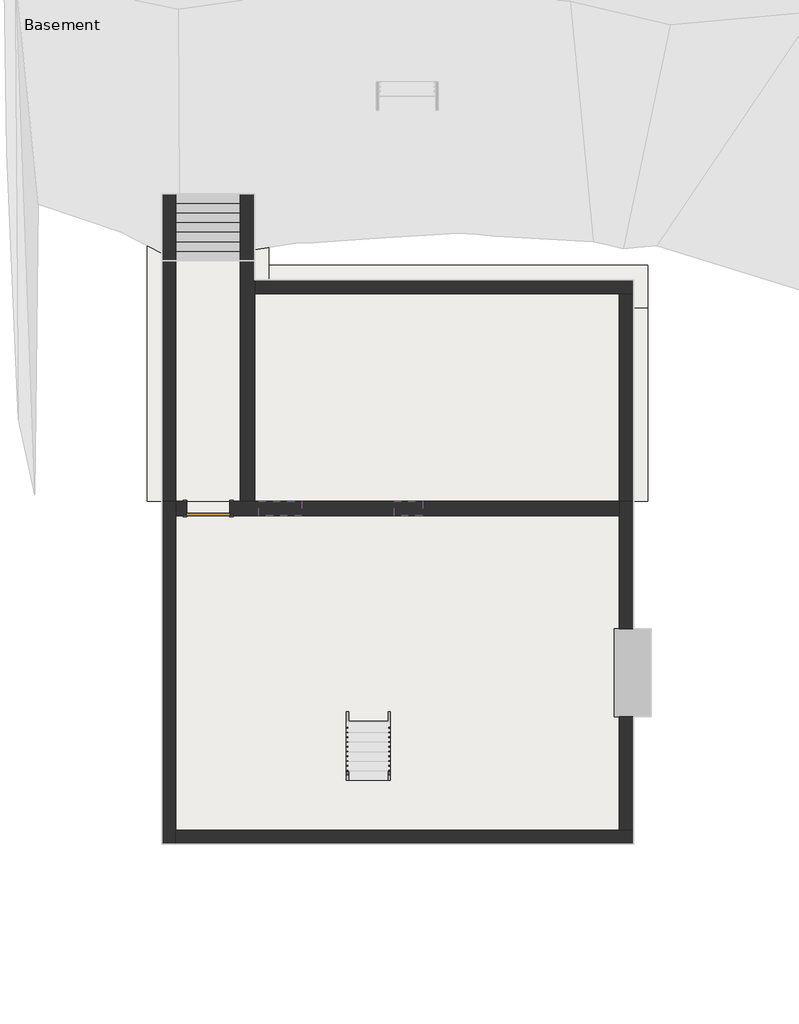
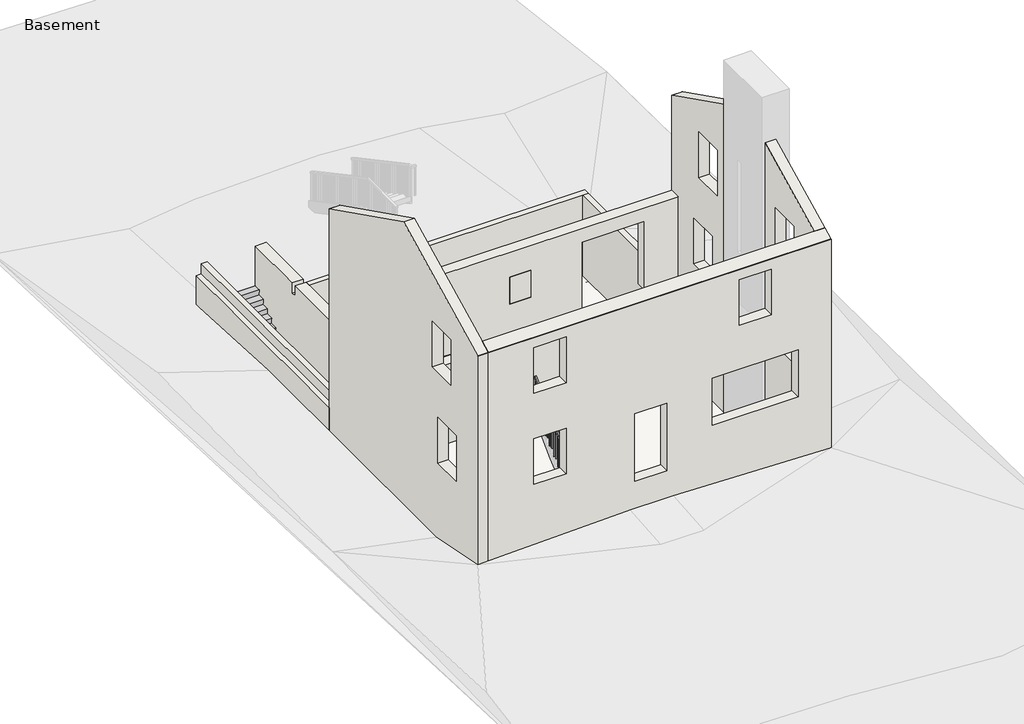
# One storey, part 1 of 2: 11 walls, 4 footings, 4 slabs, 2 railings, 1 door, 1 stair flight.
"""IFC4 building model written with IfcOpenShell, lengths in millimetres."""

import ifcopenshell
import ifcopenshell.guid

model = None  # the IFC model being written
_history = None  # IfcOwnerHistory: only IFC2X3 demands one
_inside = {}  # id of a spatial element -> (the spatial element, [elements in it])
_under = {}  # id of a project, library or spatial element -> (it, [spatial elements below it])
_declared = {}  # id of a project -> (the project, [libraries it declares])
_typed = {}  # id of a type object -> (the type object, [elements of that type])
_made_of = {}  # id of a material, layer set ... -> (it, [elements and type objects made of it])


def new_model(schema):
    """Start an empty IFC model of exactly this schema.

    Asked for "IFC4X3", IfcOpenShell would pick the latest addendum, in which some entities
    have other attributes; the version numbers below select the first issue.
    IFC2X3 requires an IfcOwnerHistory on every rooted entity: one is made here for all.
    """
    global model, _history
    if schema == "IFC4X3":
        model = ifcopenshell.file(schema_version=(4, 3, 0, 0))
    else:
        model = ifcopenshell.file(schema=schema)
    _inside.clear()
    _under.clear()
    _declared.clear()
    _typed.clear()
    _made_of.clear()
    _history = None
    if model.schema == "IFC2X3":
        org = make("IfcOrganization", Name="unknown")
        user = make(
            "IfcPersonAndOrganization",
            ThePerson=make("IfcPerson", FamilyName="unknown"),
            TheOrganization=org,
        )
        app = make(
            "IfcApplication",
            ApplicationDeveloper=org,
            Version="unknown",
            ApplicationFullName="unknown",
            ApplicationIdentifier="unknown",
        )
        _history = make(
            "IfcOwnerHistory",
            OwningUser=user,
            OwningApplication=app,
            ChangeAction="ADDED",
            CreationDate=0,
        )
    return model


def make(cls, **values):
    """One entity of the class cls with the attributes given. An attribute that is None is left unset."""
    return model.create_entity(
        cls, **{name: value for name, value in values.items() if value is not None}
    )


def rooted(cls, **values):
    """An entity with a GlobalId (a new one), such as an element, a storey or a relation."""
    return make(cls, GlobalId=ifcopenshell.guid.new(), OwnerHistory=_history, **values)


def si_unit(unit_type, name, prefix=None):
    """IfcSIUnit, for example si_unit("LENGTHUNIT", "METRE", prefix="MILLI")."""
    return make("IfcSIUnit", UnitType=unit_type, Prefix=prefix, Name=name)


def assignment(units):
    """IfcUnitAssignment: the units of a project."""
    return None if units is None else make("IfcUnitAssignment", Units=units)


def point(xyz):
    """IfcCartesianPoint."""
    return None if xyz is None else make("IfcCartesianPoint", Coordinates=xyz)


def direction(xyz):
    """IfcDirection."""
    return None if xyz is None else make("IfcDirection", DirectionRatios=xyz)


def frame(location, z_axis=None, x_axis=None):
    """IfcAxis2Placement3D, a coordinate frame: its origin and axes. An axis left out is left unset."""
    return make(
        "IfcAxis2Placement3D",
        Location=point(location),
        Axis=direction(z_axis),
        RefDirection=direction(x_axis),
    )


def origin():
    """The frame at (0, 0, 0) with its axes left unset."""
    return frame((0.0, 0.0, 0.0))


def origin_with_axes():
    """The frame at (0, 0, 0) with the z axis (0, 0, 1) and the x axis (1, 0, 0) written out."""
    return frame((0.0, 0.0, 0.0), z_axis=(0.0, 0.0, 1.0), x_axis=(1.0, 0.0, 0.0))


def place(relative_to, where):
    """IfcLocalPlacement: puts the frame where relative to a parent placement (None: the world)."""
    return make(
        "IfcLocalPlacement", PlacementRelTo=relative_to, RelativePlacement=where
    )


def context(
    kind, dimensions, precision=None, world=None, true_north=None, identifier=None
):
    """IfcGeometricRepresentationContext, for example the 3D "Model" context."""
    return make(
        "IfcGeometricRepresentationContext",
        ContextIdentifier=identifier,
        ContextType=kind,
        CoordinateSpaceDimension=dimensions,
        Precision=precision,
        WorldCoordinateSystem=world,
        TrueNorth=true_north,
    )


def project(units=None, contexts=None):
    """IfcProject with its units and contexts."""
    return rooted(
        "IfcProject",
        Name="project",
        RepresentationContexts=contexts,
        UnitsInContext=assignment(units),
    )


def spatial(cls, under=None, at=None, **own):
    """A site, building, storey or space (cls), placed at a placement, below another one or the project."""
    s = rooted(cls, ObjectPlacement=at, **own)
    if under is not None:
        _under.setdefault(under.id(), (under, []))[1].append(s)
    return s


def polyline(points):
    """IfcPolyline through the points."""
    return make("IfcPolyline", Points=[point(p) for p in points])


def outline(outer, holes=None, kind="AREA"):
    """IfcArbitraryClosedProfileDef: a profile drawn as a closed curve; with holes, ...WithVoids."""
    if holes is None:
        return make("IfcArbitraryClosedProfileDef", ProfileType=kind, OuterCurve=outer)
    return make(
        "IfcArbitraryProfileDefWithVoids",
        ProfileType=kind,
        OuterCurve=outer,
        InnerCurves=holes,
    )


def extrude(swept, where, along, depth):
    """IfcExtrudedAreaSolid: the profile swept, set in the frame where, extruded along a direction by depth."""
    return make(
        "IfcExtrudedAreaSolid",
        SweptArea=swept,
        Position=where,
        ExtrudedDirection=direction(along),
        Depth=depth,
    )


def faces_of(points, faces, orient=None, outer=None):
    """IfcFace entities. A face is a list of loops; a loop is a list of indices into points, from 0.

    orient and outer hold one flag for each loop. By default every Orientation is true, the
    first loop of a face is its IfcFaceOuterBound and the others are IfcFaceBound.
    """
    made = []
    for i, loops in enumerate(faces):
        bounds = []
        for j, loop in enumerate(loops):
            is_outer = j == 0 if outer is None else outer[i][j]
            bounds.append(
                make(
                    "IfcFaceOuterBound" if is_outer else "IfcFaceBound",
                    Bound=make("IfcPolyLoop", Polygon=[points[k] for k in loop]),
                    Orientation=True if orient is None else orient[i][j],
                )
            )
        made.append(make("IfcFace", Bounds=bounds))
    return made


def faceted_brep(points, faces, orient=None, outer=None, voids=None):
    """IfcFacetedBrep: a solid bounded by flat faces; with voids (closed shells), ...WithVoids."""
    shared = [point(p) for p in points]
    hull = make("IfcClosedShell", CfsFaces=faces_of(shared, faces, orient, outer))
    if voids is None:
        return make("IfcFacetedBrep", Outer=hull)
    return make(
        "IfcFacetedBrepWithVoids",
        Outer=hull,
        Voids=[
            make(cls, CfsFaces=faces_of(shared, fs, o, b)) for cls, fs, o, b in voids
        ],
    )


def shape(context_of_items, identifier, shape_type, items):
    """IfcShapeRepresentation: the items that make up one representation, for example the "Body"."""
    return make(
        "IfcShapeRepresentation",
        ContextOfItems=context_of_items,
        RepresentationIdentifier=identifier,
        RepresentationType=shape_type,
        Items=items,
    )


def source(mapping_origin, context_of_items, identifier, shape_type, items):
    """IfcRepresentationMap: a shape defined once, which mapped items show again and again."""
    return make(
        "IfcRepresentationMap",
        MappingOrigin=mapping_origin,
        MappedRepresentation=shape(context_of_items, identifier, shape_type, items),
    )


def transform(
    local_origin,
    x_axis=None,
    y_axis=None,
    z_axis=None,
    scale=None,
    scale2=None,
    scale3=None,
    uniform=True,
):
    """IfcCartesianTransformationOperator3D, or its non-uniform kind. x_axis, y_axis, z_axis: its Axis1, 2, 3."""
    if uniform:
        return make(
            "IfcCartesianTransformationOperator3D",
            Axis1=direction(x_axis),
            Axis2=direction(y_axis),
            LocalOrigin=point(local_origin),
            Scale=scale,
            Axis3=direction(z_axis),
        )
    return make(
        "IfcCartesianTransformationOperator3DnonUniform",
        Axis1=direction(x_axis),
        Axis2=direction(y_axis),
        LocalOrigin=point(local_origin),
        Scale=scale,
        Axis3=direction(z_axis),
        Scale2=scale2,
        Scale3=scale3,
    )


def mapped(mapping_source, mapping_target):
    """IfcMappedItem: shows the shape of a source again, moved by a transform."""
    return make(
        "IfcMappedItem", MappingSource=mapping_source, MappingTarget=mapping_target
    )


def made_of(thing, what):
    """Note that an element or type object is made of a material, layer set ...; save() writes the relation."""
    if what is not None:
        _made_of.setdefault(what.id(), (what, []))[1].append(thing)
    return thing


def element(
    cls,
    number,
    at=None,
    inside=None,
    cuts=None,
    type_object=None,
    material=None,
    context=None,
    identifier="Body",
    shape_type=None,
    held_by="IfcProductDefinitionShape",
    body=None,
    shapes=None,
    **own,
):
    """One element of the class cls, such as IfcWall. Its Tag is "e" and its number.

    at: its placement. inside: the storey or other place that contains it. cuts: it is an
    opening in that element (IfcRelVoidsElement). A single representation is given by context,
    identifier, shape_type and body (its items); several are given by shapes. held_by: the class
    of the entity that holds the representations. save() writes the other relations.
    """
    e = rooted(cls, Tag="e%d" % number, ObjectPlacement=at, **own)
    if body is not None:
        shapes = [shape(context, identifier, shape_type, body)]
    if shapes is not None:
        e.Representation = make(held_by, Representations=shapes)
    if inside is not None:
        _inside.setdefault(inside.id(), (inside, []))[1].append(e)
    if cuts is not None:
        rooted(
            "IfcRelVoidsElement", RelatingBuildingElement=cuts, RelatedOpeningElement=e
        )
    if type_object is not None:
        _typed.setdefault(type_object.id(), (type_object, []))[1].append(e)
    return made_of(e, material)


def aggregate(whole, parts):
    """IfcRelAggregates: a whole, such as a stair, and the parts it consists of."""
    return rooted("IfcRelAggregates", RelatingObject=whole, RelatedObjects=parts)


def save(model, path):
    """Write the relations noted so far, then the file.

    IfcRelAggregates (storeys below a building ...), IfcRelContainedInSpatialStructure (elements
    in a storey), IfcRelDefinesByType, IfcRelAssociatesMaterial and IfcRelDeclares: one each for
    every whole, place, type object, material and project.
    """
    for whole, parts in _under.values():
        aggregate(whole, parts)
    for where, things in _inside.values():
        rooted(
            "IfcRelContainedInSpatialStructure",
            RelatedElements=things,
            RelatingStructure=where,
        )
    for kind, things in _typed.values():
        rooted("IfcRelDefinesByType", RelatedObjects=things, RelatingType=kind)
    for what, things in _made_of.values():
        rooted("IfcRelAssociatesMaterial", RelatedObjects=things, RelatingMaterial=what)
    for by, libraries in _declared.values():
        rooted("IfcRelDeclares", RelatingContext=by, RelatedDefinitions=libraries)
    model.write(path)


def door_03272193(model_context):
    return source(origin(), model_context, "Body", "SweptSolid", [
        extrude(outline(polyline([(2209.8, -533.4), (0.0, -533.4), (0.0, -457.2), (2133.6, -457.2), (2133.6, 457.2), (0.0, 457.2), (0.0, 533.4), (2209.8, 533.4), (2209.8, -533.4)])), frame((0.0, 152.4, 0.0), z_axis=(0.0, 1.0, 0.0), x_axis=(0.0, 0.0, 1.0)), (0.0, 0.0, 1.0), 25.4),
        extrude(outline(polyline([(2209.8, 533.4), (2209.8, -533.4), (0.0, -533.4), (0.0, -457.2), (2133.6, -457.2), (2133.6, 457.2), (0.0, 457.2), (0.0, 533.4), (2209.8, 533.4)])), frame((0.0, -177.8, 0.0), z_axis=(0.0, 1.0, 0.0), x_axis=(0.0, 0.0, 1.0)), (0.0, 0.0, 1.0), 25.4),
        extrude(outline(polyline([(457.2, 101.6), (-457.2, 101.6), (-457.2, 152.4), (457.2, 152.4), (457.2, 101.6)])), origin_with_axes(), (0.0, 0.0, 1.0), 2133.6),
    ])


model = new_model("IFC4")

# Units and contexts
model_context = context("Model", 3, world=origin())
ifc_project = project(units=[si_unit("LENGTHUNIT", "METRE", prefix="MILLI")], contexts=[model_context])

# Site, building, storey
site = spatial("IfcSite", under=ifc_project)
building = spatial("IfcBuilding", under=site)
storey = spatial("IfcBuildingStorey", under=building, Name="Basement", Elevation=-2667.0)

# Door
placement = place(None, origin())
door_shape = door_03272193(model_context)
element("IfcDoor", 1, ObjectType="Single-Flush : 36\" x 84\"", at=placement, inside=storey, context=model_context, shape_type="MappedRepresentation", body=[
    mapped(door_shape, transform((-4998.5803068, 2999.6888758, -2667.0), x_axis=(-1.0, 0.0, 0.0), y_axis=(0.0, -1.0, 0.0), z_axis=(0.0, 0.0, 1.0))),
])

# Footings
element("IfcFooting", 2, ObjectType="Bearing Footing - 36\" x 12\"", at=placement, inside=storey, context=model_context, shape_type="SweptSolid", body=[
    extrude(outline(polyline([(-5379.5803068, 3152.0888758), (-6293.9803068, 3152.0888758), (-6293.9803068, 10010.0888758), (-5379.5803068, 10010.0888758), (-5379.5803068, 3152.0888758)])), frame((0.0, 0.0, -3073.4), z_axis=(0.0, 0.0, 1.0), x_axis=(1.0, 0.0, 0.0)), (0.0, 0.0, 1.0), 304.8),
])
element("IfcFooting", 3, ObjectType="Bearing Footing - 36\" x 12\"", at=placement, inside=storey, context=model_context, shape_type="Brep", body=[
    faceted_brep([(-3703.1803068, 7266.8888758, -2768.6), (3459.6196932, 7266.8888758, -2768.6), (4374.0196932, 7266.8888758, -2768.6), (4374.0196932, 8181.2888758, -2768.6), (-3703.1803068, 8181.2888758, -2768.6), (-3703.1803068, 8181.2888758, -3073.4), (4374.0196932, 8181.2888758, -3073.4), (-3703.1803068, 7266.8888758, -3073.4), (4374.0196932, 7266.8888758, -3073.4), (3459.6196932, 7266.8888758, -3073.4)], [[[0, 1, 2, 3, 4]], [[5, 4, 3, 6]], [[7, 5, 6, 8, 9]], [[0, 7, 9, 8, 2, 1]], [[0, 4, 5, 7]], [[3, 2, 8, 6]]]),
])
element("IfcFooting", 4, ObjectType="Bearing Footing - 36\" x 12\"", at=placement, inside=storey, context=model_context, shape_type="SweptSolid", body=[
    extrude(outline(polyline([(4374.0196932, 3152.0888758), (3459.6196932, 3152.0888758), (3459.6196932, 7266.8888758), (4374.0196932, 7266.8888758), (4374.0196932, 3152.0888758)])), frame((0.0, 0.0, -3073.4), z_axis=(0.0, 0.0, 1.0), x_axis=(1.0, 0.0, 0.0)), (0.0, 0.0, 1.0), 304.8),
])
element("IfcFooting", 5, ObjectType="Bearing Footing - 36\" x 12\"", at=placement, inside=storey, context=model_context, shape_type="Brep", body=[
    faceted_brep([(-3703.1803068, 3152.0888758, -2768.6), (-4617.5803068, 3152.0888758, -2768.6), (-4617.5803068, 3152.0888758, -3073.4), (-3703.1803068, 3152.0888758, -3073.4), (-4617.5803068, 10010.0888758, -2768.6), (-3703.1803068, 10010.0888758, -2768.6), (-3703.1803068, 10010.0888758, -3073.4), (-4617.5803068, 10010.0888758, -3073.4), (-3703.1803068, 7266.8888758, -2768.6), (-3703.1803068, 8181.2888758, -2768.6), (-3703.1803068, 8181.2888758, -3073.4), (-3703.1803068, 7266.8888758, -3073.4)], [[[0, 1, 2, 3]], [[4, 5, 6, 7]], [[0, 8, 9, 5, 4, 1]], [[2, 1, 4, 7]], [[3, 2, 7, 6, 10, 11]], [[0, 3, 11, 10, 6, 5, 9, 8]]]),
])

# Railings
element("IfcRailing", 6, ObjectType="Handrail - Rectangular", at=placement, inside=storey, context=model_context, shape_type="SweptSolid", body=[
    extrude(outline(polyline([(-2791.5111242, -1631.7331862), (-2791.5111242, -1562.1), (-149.9111242, 914.4), (-149.9111242, 844.7668138), (-2791.5111242, -1631.7331862)])), frame((-1163.1803068, 0.0, 0.0), z_axis=(1.0, 0.0, 0.0), x_axis=(0.0, 1.0, 0.0)), (0.0, 0.0, 1.0), 50.8),
    extrude(outline(polyline([(-261.0361242, 740.5871263), (-241.9861242, 758.4465013), (-241.9861242, -190.5), (-261.0361242, -190.5), (-261.0361242, 740.5871263)])), frame((-1147.3053068, 0.0, 0.0), z_axis=(1.0, 0.0, 0.0), x_axis=(0.0, 1.0, 0.0)), (0.0, 0.0, 1.0), 19.05),
    extrude(outline(polyline([(-362.6361242, 645.3371263), (-343.5861242, 663.1965013), (-343.5861242, -190.5), (-362.6361242, -190.5), (-362.6361242, 645.3371263)])), frame((-1147.3053068, 0.0, 0.0), z_axis=(1.0, 0.0, 0.0), x_axis=(0.0, 1.0, 0.0)), (0.0, 0.0, 1.0), 19.05),
    extrude(outline(polyline([(-464.2361242, 550.0871263), (-445.1861242, 567.9465013), (-445.1861242, -381.0), (-464.2361242, -381.0), (-464.2361242, 550.0871263)])), frame((-1147.3053068, 0.0, 0.0), z_axis=(1.0, 0.0, 0.0), x_axis=(0.0, 1.0, 0.0)), (0.0, 0.0, 1.0), 19.05),
    extrude(outline(polyline([(-565.8361242, 454.8371263), (-546.7861242, 472.6965013), (-546.7861242, -381.0), (-565.8361242, -381.0), (-565.8361242, 454.8371263)])), frame((-1147.3053068, 0.0, 0.0), z_axis=(1.0, 0.0, 0.0), x_axis=(0.0, 1.0, 0.0)), (0.0, 0.0, 1.0), 19.05),
    extrude(outline(polyline([(-667.4361242, 359.5871263), (-648.3861242, 377.4465013), (-648.3861242, -571.5), (-667.4361242, -571.5), (-667.4361242, 359.5871263)])), frame((-1147.3053068, 0.0, 0.0), z_axis=(1.0, 0.0, 0.0), x_axis=(0.0, 1.0, 0.0)), (0.0, 0.0, 1.0), 19.05),
    extrude(outline(polyline([(-769.0361242, 264.3371263), (-749.9861242, 282.1965013), (-749.9861242, -571.5), (-769.0361242, -571.5), (-769.0361242, 264.3371263)])), frame((-1147.3053068, 0.0, 0.0), z_axis=(1.0, 0.0, 0.0), x_axis=(0.0, 1.0, 0.0)), (0.0, 0.0, 1.0), 19.05),
    extrude(outline(polyline([(-870.6361242, 169.0871263), (-851.5861242, 186.9465013), (-851.5861242, -762.0), (-870.6361242, -762.0), (-870.6361242, 169.0871263)])), frame((-1147.3053068, 0.0, 0.0), z_axis=(1.0, 0.0, 0.0), x_axis=(0.0, 1.0, 0.0)), (0.0, 0.0, 1.0), 19.05),
    extrude(outline(polyline([(-972.2361242, 73.8371263), (-953.1861242, 91.6965013), (-953.1861242, -762.0), (-972.2361242, -762.0), (-972.2361242, 73.8371263)])), frame((-1147.3053068, 0.0, 0.0), z_axis=(1.0, 0.0, 0.0), x_axis=(0.0, 1.0, 0.0)), (0.0, 0.0, 1.0), 19.05),
    extrude(outline(polyline([(-1073.8361242, -21.4128737), (-1054.7861242, -3.5534987), (-1054.7861242, -952.5), (-1073.8361242, -952.5), (-1073.8361242, -21.4128737)])), frame((-1147.3053068, 0.0, 0.0), z_axis=(1.0, 0.0, 0.0), x_axis=(0.0, 1.0, 0.0)), (0.0, 0.0, 1.0), 19.05),
    extrude(outline(polyline([(-1175.4361242, -116.6628737), (-1156.3861242, -98.8034987), (-1156.3861242, -952.5), (-1175.4361242, -952.5), (-1175.4361242, -116.6628737)])), frame((-1147.3053068, 0.0, 0.0), z_axis=(1.0, 0.0, 0.0), x_axis=(0.0, 1.0, 0.0)), (0.0, 0.0, 1.0), 19.05),
    extrude(outline(polyline([(-1277.0361242, -211.9128737), (-1257.9861242, -194.0534987), (-1257.9861242, -1143.0), (-1277.0361242, -1143.0), (-1277.0361242, -211.9128737)])), frame((-1147.3053068, 0.0, 0.0), z_axis=(1.0, 0.0, 0.0), x_axis=(0.0, 1.0, 0.0)), (0.0, 0.0, 1.0), 19.05),
    extrude(outline(polyline([(-1378.6361242, -307.1628737), (-1359.5861242, -289.3034987), (-1359.5861242, -1143.0), (-1378.6361242, -1143.0), (-1378.6361242, -307.1628737)])), frame((-1147.3053068, 0.0, 0.0), z_axis=(1.0, 0.0, 0.0), x_axis=(0.0, 1.0, 0.0)), (0.0, 0.0, 1.0), 19.05),
    extrude(outline(polyline([(-1480.2361242, -402.4128737), (-1461.1861242, -384.5534987), (-1461.1861242, -1333.5), (-1480.2361242, -1333.5), (-1480.2361242, -402.4128737)])), frame((-1147.3053068, 0.0, 0.0), z_axis=(1.0, 0.0, 0.0), x_axis=(0.0, 1.0, 0.0)), (0.0, 0.0, 1.0), 19.05),
    extrude(outline(polyline([(-1581.8361242, -497.6628737), (-1562.7861242, -479.8034987), (-1562.7861242, -1333.5), (-1581.8361242, -1333.5), (-1581.8361242, -497.6628737)])), frame((-1147.3053068, 0.0, 0.0), z_axis=(1.0, 0.0, 0.0), x_axis=(0.0, 1.0, 0.0)), (0.0, 0.0, 1.0), 19.05),
    extrude(outline(polyline([(-1683.4361242, -592.9128737), (-1664.3861242, -575.0534987), (-1664.3861242, -1524.0), (-1683.4361242, -1524.0), (-1683.4361242, -592.9128737)])), frame((-1147.3053068, 0.0, 0.0), z_axis=(1.0, 0.0, 0.0), x_axis=(0.0, 1.0, 0.0)), (0.0, 0.0, 1.0), 19.05),
    extrude(outline(polyline([(-1785.0361242, -688.1628737), (-1765.9861242, -670.3034987), (-1765.9861242, -1524.0), (-1785.0361242, -1524.0), (-1785.0361242, -688.1628737)])), frame((-1147.3053068, 0.0, 0.0), z_axis=(1.0, 0.0, 0.0), x_axis=(0.0, 1.0, 0.0)), (0.0, 0.0, 1.0), 19.05),
    extrude(outline(polyline([(-1886.6361242, -783.4128737), (-1867.5861242, -765.5534987), (-1867.5861242, -1714.5), (-1886.6361242, -1714.5), (-1886.6361242, -783.4128737)])), frame((-1147.3053068, 0.0, 0.0), z_axis=(1.0, 0.0, 0.0), x_axis=(0.0, 1.0, 0.0)), (0.0, 0.0, 1.0), 19.05),
    extrude(outline(polyline([(-1988.2361242, -878.6628737), (-1969.1861242, -860.8034987), (-1969.1861242, -1714.5), (-1988.2361242, -1714.5), (-1988.2361242, -878.6628737)])), frame((-1147.3053068, 0.0, 0.0), z_axis=(1.0, 0.0, 0.0), x_axis=(0.0, 1.0, 0.0)), (0.0, 0.0, 1.0), 19.05),
    extrude(outline(polyline([(-2089.8361242, -973.9128737), (-2070.7861242, -956.0534987), (-2070.7861242, -1905.0), (-2089.8361242, -1905.0), (-2089.8361242, -973.9128737)])), frame((-1147.3053068, 0.0, 0.0), z_axis=(1.0, 0.0, 0.0), x_axis=(0.0, 1.0, 0.0)), (0.0, 0.0, 1.0), 19.05),
    extrude(outline(polyline([(-2191.4361242, -1069.1628737), (-2172.3861242, -1051.3034987), (-2172.3861242, -1905.0), (-2191.4361242, -1905.0), (-2191.4361242, -1069.1628737)])), frame((-1147.3053068, 0.0, 0.0), z_axis=(1.0, 0.0, 0.0), x_axis=(0.0, 1.0, 0.0)), (0.0, 0.0, 1.0), 19.05),
    extrude(outline(polyline([(-2293.0361242, -1164.4128737), (-2273.9861242, -1146.5534987), (-2273.9861242, -2095.5), (-2293.0361242, -2095.5), (-2293.0361242, -1164.4128737)])), frame((-1147.3053068, 0.0, 0.0), z_axis=(1.0, 0.0, 0.0), x_axis=(0.0, 1.0, 0.0)), (0.0, 0.0, 1.0), 19.05),
    extrude(outline(polyline([(-2394.6361242, -1259.6628737), (-2375.5861242, -1241.8034987), (-2375.5861242, -2095.5), (-2394.6361242, -2095.5), (-2394.6361242, -1259.6628737)])), frame((-1147.3053068, 0.0, 0.0), z_axis=(1.0, 0.0, 0.0), x_axis=(0.0, 1.0, 0.0)), (0.0, 0.0, 1.0), 19.05),
    extrude(outline(polyline([(-2496.2361242, -1354.9128737), (-2477.1861242, -1337.0534987), (-2477.1861242, -2286.0), (-2496.2361242, -2286.0), (-2496.2361242, -1354.9128737)])), frame((-1147.3053068, 0.0, 0.0), z_axis=(1.0, 0.0, 0.0), x_axis=(0.0, 1.0, 0.0)), (0.0, 0.0, 1.0), 19.05),
    extrude(outline(polyline([(-2597.8361242, -1450.1628737), (-2578.7861242, -1432.3034987), (-2578.7861242, -2286.0), (-2597.8361242, -2286.0), (-2597.8361242, -1450.1628737)])), frame((-1147.3053068, 0.0, 0.0), z_axis=(1.0, 0.0, 0.0), x_axis=(0.0, 1.0, 0.0)), (0.0, 0.0, 1.0), 19.05),
    extrude(outline(polyline([(-2699.4361242, -1545.4128737), (-2680.3861242, -1527.5534987), (-2680.3861242, -2476.5), (-2699.4361242, -2476.5), (-2699.4361242, -1545.4128737)])), frame((-1147.3053068, 0.0, 0.0), z_axis=(1.0, 0.0, 0.0), x_axis=(0.0, 1.0, 0.0)), (0.0, 0.0, 1.0), 19.05),
    extrude(outline(polyline([(-168.9611242, 826.9074388), (-149.9111242, 844.7668138), (-149.9111242, -190.5), (-168.9611242, -190.5), (-168.9611242, 826.9074388)])), frame((-1147.3053068, 0.0, 0.0), z_axis=(1.0, 0.0, 0.0), x_axis=(0.0, 1.0, 0.0)), (0.0, 0.0, 1.0), 19.05),
    extrude(outline(polyline([(-2791.5111242, -1631.7331862), (-2772.4611242, -1613.8738112), (-2772.4611242, -2476.5), (-2791.5111242, -2476.5), (-2791.5111242, -1631.7331862)])), frame((-1147.3053068, 0.0, 0.0), z_axis=(1.0, 0.0, 0.0), x_axis=(0.0, 1.0, 0.0)), (0.0, 0.0, 1.0), 19.05),
])
element("IfcRailing", 7, ObjectType="Handrail - Rectangular", at=placement, inside=storey, context=model_context, shape_type="SweptSolid", body=[
    extrude(outline(polyline([(-2791.5111242, -1631.7331862), (-2791.5111242, -1562.1), (-149.9111242, 914.4), (-149.9111242, 844.7668138), (-2791.5111242, -1631.7331862)])), frame((-2052.1803068, 0.0, 0.0), z_axis=(1.0, 0.0, 0.0), x_axis=(0.0, 1.0, 0.0)), (0.0, 0.0, 1.0), 50.8),
    extrude(outline(polyline([(-241.9861242, 758.4465013), (-241.9861242, -190.5), (-261.0361242, -190.5), (-261.0361242, 740.5871263), (-241.9861242, 758.4465013)])), frame((-2036.3053068, 0.0, 0.0), z_axis=(1.0, 0.0, 0.0), x_axis=(0.0, 1.0, 0.0)), (0.0, 0.0, 1.0), 19.05),
    extrude(outline(polyline([(-343.5861242, 663.1965013), (-343.5861242, -190.5), (-362.6361242, -190.5), (-362.6361242, 645.3371263), (-343.5861242, 663.1965013)])), frame((-2036.3053068, 0.0, 0.0), z_axis=(1.0, 0.0, 0.0), x_axis=(0.0, 1.0, 0.0)), (0.0, 0.0, 1.0), 19.05),
    extrude(outline(polyline([(-445.1861242, 567.9465013), (-445.1861242, -381.0), (-464.2361242, -381.0), (-464.2361242, 550.0871263), (-445.1861242, 567.9465013)])), frame((-2036.3053068, 0.0, 0.0), z_axis=(1.0, 0.0, 0.0), x_axis=(0.0, 1.0, 0.0)), (0.0, 0.0, 1.0), 19.05),
    extrude(outline(polyline([(-546.7861242, 472.6965013), (-546.7861242, -381.0), (-565.8361242, -381.0), (-565.8361242, 454.8371263), (-546.7861242, 472.6965013)])), frame((-2036.3053068, 0.0, 0.0), z_axis=(1.0, 0.0, 0.0), x_axis=(0.0, 1.0, 0.0)), (0.0, 0.0, 1.0), 19.05),
    extrude(outline(polyline([(-648.3861242, 377.4465013), (-648.3861242, -571.5), (-667.4361242, -571.5), (-667.4361242, 359.5871263), (-648.3861242, 377.4465013)])), frame((-2036.3053068, 0.0, 0.0), z_axis=(1.0, 0.0, 0.0), x_axis=(0.0, 1.0, 0.0)), (0.0, 0.0, 1.0), 19.05),
    extrude(outline(polyline([(-749.9861242, 282.1965013), (-749.9861242, -571.5), (-769.0361242, -571.5), (-769.0361242, 264.3371263), (-749.9861242, 282.1965013)])), frame((-2036.3053068, 0.0, 0.0), z_axis=(1.0, 0.0, 0.0), x_axis=(0.0, 1.0, 0.0)), (0.0, 0.0, 1.0), 19.05),
    extrude(outline(polyline([(-851.5861242, 186.9465013), (-851.5861242, -762.0), (-870.6361242, -762.0), (-870.6361242, 169.0871263), (-851.5861242, 186.9465013)])), frame((-2036.3053068, 0.0, 0.0), z_axis=(1.0, 0.0, 0.0), x_axis=(0.0, 1.0, 0.0)), (0.0, 0.0, 1.0), 19.05),
    extrude(outline(polyline([(-953.1861242, 91.6965013), (-953.1861242, -762.0), (-972.2361242, -762.0), (-972.2361242, 73.8371263), (-953.1861242, 91.6965013)])), frame((-2036.3053068, 0.0, 0.0), z_axis=(1.0, 0.0, 0.0), x_axis=(0.0, 1.0, 0.0)), (0.0, 0.0, 1.0), 19.05),
    extrude(outline(polyline([(-1054.7861242, -3.5534987), (-1054.7861242, -952.5), (-1073.8361242, -952.5), (-1073.8361242, -21.4128737), (-1054.7861242, -3.5534987)])), frame((-2036.3053068, 0.0, 0.0), z_axis=(1.0, 0.0, 0.0), x_axis=(0.0, 1.0, 0.0)), (0.0, 0.0, 1.0), 19.05),
    extrude(outline(polyline([(-1156.3861242, -98.8034987), (-1156.3861242, -952.5), (-1175.4361242, -952.5), (-1175.4361242, -116.6628737), (-1156.3861242, -98.8034987)])), frame((-2036.3053068, 0.0, 0.0), z_axis=(1.0, 0.0, 0.0), x_axis=(0.0, 1.0, 0.0)), (0.0, 0.0, 1.0), 19.05),
    extrude(outline(polyline([(-1257.9861242, -194.0534987), (-1257.9861242, -1143.0), (-1277.0361242, -1143.0), (-1277.0361242, -211.9128737), (-1257.9861242, -194.0534987)])), frame((-2036.3053068, 0.0, 0.0), z_axis=(1.0, 0.0, 0.0), x_axis=(0.0, 1.0, 0.0)), (0.0, 0.0, 1.0), 19.05),
    extrude(outline(polyline([(-1359.5861242, -289.3034987), (-1359.5861242, -1143.0), (-1378.6361242, -1143.0), (-1378.6361242, -307.1628737), (-1359.5861242, -289.3034987)])), frame((-2036.3053068, 0.0, 0.0), z_axis=(1.0, 0.0, 0.0), x_axis=(0.0, 1.0, 0.0)), (0.0, 0.0, 1.0), 19.05),
    extrude(outline(polyline([(-1461.1861242, -384.5534987), (-1461.1861242, -1333.5), (-1480.2361242, -1333.5), (-1480.2361242, -402.4128737), (-1461.1861242, -384.5534987)])), frame((-2036.3053068, 0.0, 0.0), z_axis=(1.0, 0.0, 0.0), x_axis=(0.0, 1.0, 0.0)), (0.0, 0.0, 1.0), 19.05),
    extrude(outline(polyline([(-1562.7861242, -479.8034987), (-1562.7861242, -1333.5), (-1581.8361242, -1333.5), (-1581.8361242, -497.6628737), (-1562.7861242, -479.8034987)])), frame((-2036.3053068, 0.0, 0.0), z_axis=(1.0, 0.0, 0.0), x_axis=(0.0, 1.0, 0.0)), (0.0, 0.0, 1.0), 19.05),
    extrude(outline(polyline([(-1664.3861242, -575.0534987), (-1664.3861242, -1524.0), (-1683.4361242, -1524.0), (-1683.4361242, -592.9128737), (-1664.3861242, -575.0534987)])), frame((-2036.3053068, 0.0, 0.0), z_axis=(1.0, 0.0, 0.0), x_axis=(0.0, 1.0, 0.0)), (0.0, 0.0, 1.0), 19.05),
    extrude(outline(polyline([(-1765.9861242, -670.3034987), (-1765.9861242, -1524.0), (-1785.0361242, -1524.0), (-1785.0361242, -688.1628737), (-1765.9861242, -670.3034987)])), frame((-2036.3053068, 0.0, 0.0), z_axis=(1.0, 0.0, 0.0), x_axis=(0.0, 1.0, 0.0)), (0.0, 0.0, 1.0), 19.05),
    extrude(outline(polyline([(-1867.5861242, -765.5534987), (-1867.5861242, -1714.5), (-1886.6361242, -1714.5), (-1886.6361242, -783.4128737), (-1867.5861242, -765.5534987)])), frame((-2036.3053068, 0.0, 0.0), z_axis=(1.0, 0.0, 0.0), x_axis=(0.0, 1.0, 0.0)), (0.0, 0.0, 1.0), 19.05),
    extrude(outline(polyline([(-1969.1861242, -860.8034987), (-1969.1861242, -1714.5), (-1988.2361242, -1714.5), (-1988.2361242, -878.6628737), (-1969.1861242, -860.8034987)])), frame((-2036.3053068, 0.0, 0.0), z_axis=(1.0, 0.0, 0.0), x_axis=(0.0, 1.0, 0.0)), (0.0, 0.0, 1.0), 19.05),
    extrude(outline(polyline([(-2070.7861242, -956.0534987), (-2070.7861242, -1905.0), (-2089.8361242, -1905.0), (-2089.8361242, -973.9128737), (-2070.7861242, -956.0534987)])), frame((-2036.3053068, 0.0, 0.0), z_axis=(1.0, 0.0, 0.0), x_axis=(0.0, 1.0, 0.0)), (0.0, 0.0, 1.0), 19.05),
    extrude(outline(polyline([(-2172.3861242, -1051.3034987), (-2172.3861242, -1905.0), (-2191.4361242, -1905.0), (-2191.4361242, -1069.1628737), (-2172.3861242, -1051.3034987)])), frame((-2036.3053068, 0.0, 0.0), z_axis=(1.0, 0.0, 0.0), x_axis=(0.0, 1.0, 0.0)), (0.0, 0.0, 1.0), 19.05),
    extrude(outline(polyline([(-2273.9861242, -1146.5534987), (-2273.9861242, -2095.5), (-2293.0361242, -2095.5), (-2293.0361242, -1164.4128737), (-2273.9861242, -1146.5534987)])), frame((-2036.3053068, 0.0, 0.0), z_axis=(1.0, 0.0, 0.0), x_axis=(0.0, 1.0, 0.0)), (0.0, 0.0, 1.0), 19.05),
    extrude(outline(polyline([(-2375.5861242, -1241.8034987), (-2375.5861242, -2095.5), (-2394.6361242, -2095.5), (-2394.6361242, -1259.6628737), (-2375.5861242, -1241.8034987)])), frame((-2036.3053068, 0.0, 0.0), z_axis=(1.0, 0.0, 0.0), x_axis=(0.0, 1.0, 0.0)), (0.0, 0.0, 1.0), 19.05),
    extrude(outline(polyline([(-2477.1861242, -1337.0534987), (-2477.1861242, -2286.0), (-2496.2361242, -2286.0), (-2496.2361242, -1354.9128737), (-2477.1861242, -1337.0534987)])), frame((-2036.3053068, 0.0, 0.0), z_axis=(1.0, 0.0, 0.0), x_axis=(0.0, 1.0, 0.0)), (0.0, 0.0, 1.0), 19.05),
    extrude(outline(polyline([(-2578.7861242, -1432.3034987), (-2578.7861242, -2286.0), (-2597.8361242, -2286.0), (-2597.8361242, -1450.1628737), (-2578.7861242, -1432.3034987)])), frame((-2036.3053068, 0.0, 0.0), z_axis=(1.0, 0.0, 0.0), x_axis=(0.0, 1.0, 0.0)), (0.0, 0.0, 1.0), 19.05),
    extrude(outline(polyline([(-2680.3861242, -1527.5534987), (-2680.3861242, -2476.5), (-2699.4361242, -2476.5), (-2699.4361242, -1545.4128737), (-2680.3861242, -1527.5534987)])), frame((-2036.3053068, 0.0, 0.0), z_axis=(1.0, 0.0, 0.0), x_axis=(0.0, 1.0, 0.0)), (0.0, 0.0, 1.0), 19.05),
    extrude(outline(polyline([(-149.9111242, 844.7668138), (-149.9111242, -190.5), (-168.9611242, -190.5), (-168.9611242, 826.9074388), (-149.9111242, 844.7668138)])), frame((-2036.3053068, 0.0, 0.0), z_axis=(1.0, 0.0, 0.0), x_axis=(0.0, 1.0, 0.0)), (0.0, 0.0, 1.0), 19.05),
    extrude(outline(polyline([(-2772.4611242, -1613.8738112), (-2772.4611242, -2476.5), (-2791.5111242, -2476.5), (-2791.5111242, -1631.7331862), (-2772.4611242, -1613.8738112)])), frame((-2036.3053068, 0.0, 0.0), z_axis=(1.0, 0.0, 0.0), x_axis=(0.0, 1.0, 0.0)), (0.0, 0.0, 1.0), 19.05),
])

# Slabs
element("IfcSlab", 8, ObjectType="4\" Concrete", at=placement, inside=storey, context=model_context, shape_type="SweptSolid", body=[
    extrude(outline(polyline([(-5684.3803068, 8384.4888758), (-4312.7803068, 8384.4888758), (-4312.7803068, 3152.0888758), (-5684.3803068, 3152.0888758), (-5684.3803068, 8384.4888758)])), frame((0.0, 0.0, -2768.6), z_axis=(0.0, 0.0, 1.0), x_axis=(1.0, 0.0, 0.0)), (0.0, 0.0, 1.0), 101.6),
])
element("IfcSlab", 9, ObjectType="Pad 1", at=placement, inside=storey, context=model_context, shape_type="SweptSolid", body=[
    extrude(outline(polyline([(4069.2196932, 434.2888758), (4450.2196932, 434.2888758), (4450.2196932, -1445.3111242), (4069.2196932, -1445.3111242), (4069.2196932, -4163.1111242), (-5989.1803068, -4163.1111242), (-5989.1803068, 3152.0888758), (4069.2196932, 3152.0888758), (4069.2196932, 434.2888758)])), frame((0.0, 0.0, -2774.95), z_axis=(0.0, 0.0, 1.0), x_axis=(1.0, 0.0, 0.0)), (0.0, 0.0, 1.0), 6.35),
])
element("IfcSlab", 10, ObjectType="Pad 1", at=placement, inside=storey, context=model_context, shape_type="SweptSolid", body=[
    extrude(outline(polyline([(-5989.1803068, 8275.4102719), (-4007.9803068, 8275.4102719), (-4007.9803068, 7876.4888758), (4069.2196932, 7876.4888758), (4069.2196932, 3152.0888758), (-5989.1803068, 3152.0888758), (-5989.1803068, 8275.4102719)])), frame((0.0, 0.0, -2774.95), z_axis=(0.0, 0.0, 1.0), x_axis=(1.0, 0.0, 0.0)), (0.0, 0.0, 1.0), 6.35),
])
element("IfcSlab", 11, ObjectType="Pad 1", at=placement, inside=storey, context=model_context, shape_type="SweptSolid", body=[
    extrude(outline(polyline([(9705.2888758, -1653.200634), (8275.4102719, -2776.6756068), (8275.4102719, -2768.6), (9705.2888758, -1645.1250272), (9705.2888758, -1653.200634)])), frame((-5989.1803068, 0.0, 0.0), z_axis=(1.0, 0.0, 0.0), x_axis=(0.0, 1.0, 0.0)), (0.0, 0.0, 1.0), 1981.2),
])

# Stair flight
element("IfcStairFlight", 12, ObjectType="3/4\" Nosing", at=placement, inside=storey, context=model_context, shape_type="Brep", body=[
    faceted_brep([(-4312.7803068, 8282.8888758, -2507.3428571), (-5684.3803068, 8282.8888758, -2507.3428571), (-5684.3803068, 8301.9388758, -2667.0), (-4312.7803068, 8301.9388758, -2667.0), (-4312.7803068, 8505.1388758, -2507.3428571), (-5684.3803068, 8505.1388758, -2507.3428571), (-5684.3803068, 8505.1388758, -2588.0989541), (-5684.3803068, 8404.7193628, -2667.0), (-4312.7803068, 8404.7193628, -2667.0), (-4312.7803068, 8505.1388758, -2588.0989541), (-5684.3803068, 8486.0888758, -2347.6857143), (-4312.7803068, 8486.0888758, -2347.6857143), (-4312.7803068, 8708.3388758, -2347.6857143), (-5684.3803068, 8708.3388758, -2347.6857143), (-5684.3803068, 8708.3388758, -2428.4418112), (-4312.7803068, 8708.3388758, -2428.4418112), (-5684.3803068, 8689.2888758, -2188.0285714), (-4312.7803068, 8689.2888758, -2188.0285714), (-4312.7803068, 8911.5388758, -2188.0285714), (-5684.3803068, 8911.5388758, -2188.0285714), (-5684.3803068, 8911.5388758, -2268.7846684), (-4312.7803068, 8911.5388758, -2268.7846684), (-5684.3803068, 8892.4888758, -2028.3714286), (-4312.7803068, 8892.4888758, -2028.3714286), (-4312.7803068, 9114.7388758, -2028.3714286), (-5684.3803068, 9114.7388758, -2028.3714286), (-5684.3803068, 9114.7388758, -2109.1275255), (-4312.7803068, 9114.7388758, -2109.1275255), (-5684.3803068, 9095.6888758, -1868.7142857), (-4312.7803068, 9095.6888758, -1868.7142857), (-4312.7803068, 9317.9388758, -1868.7142857), (-5684.3803068, 9317.9388758, -1868.7142857), (-5684.3803068, 9317.9388758, -1949.4703827), (-4312.7803068, 9317.9388758, -1949.4703827), (-5684.3803068, 9298.8888758, -1709.0571429), (-4312.7803068, 9298.8888758, -1709.0571429), (-4312.7803068, 9521.1388758, -1709.0571429), (-5684.3803068, 9521.1388758, -1709.0571429), (-5684.3803068, 9521.1388758, -1789.8132398), (-4312.7803068, 9521.1388758, -1789.8132398), (-5684.3803068, 9705.2888758, -1645.1239541), (-4312.7803068, 9705.2888758, -1645.1239541), (-5684.3803068, 9502.0888758, -1549.4), (-4312.7803068, 9502.0888758, -1549.4), (-4312.7803068, 9705.2888758, -1549.4), (-5684.3803068, 9705.2888758, -1549.4)], [[[0, 1, 2, 3]], [[1, 0, 4, 5]], [[1, 5, 6, 7, 2]], [[4, 0, 3, 8, 9]], [[10, 11, 12, 13]], [[10, 13, 14, 6, 5]], [[12, 11, 4, 9, 15]], [[5, 4, 11, 10]], [[16, 17, 18, 19]], [[16, 19, 20, 14, 13]], [[18, 17, 12, 15, 21]], [[13, 12, 17, 16]], [[22, 23, 24, 25]], [[22, 25, 26, 20, 19]], [[24, 23, 18, 21, 27]], [[19, 18, 23, 22]], [[28, 29, 30, 31]], [[28, 31, 32, 26, 25]], [[30, 29, 24, 27, 33]], [[25, 24, 29, 28]], [[34, 35, 36, 37]], [[34, 37, 38, 32, 31]], [[36, 35, 30, 33, 39]], [[31, 30, 35, 34]], [[3, 2, 7, 8]], [[8, 7, 6, 14, 20, 26, 32, 38, 40, 41, 39, 33, 27, 21, 15, 9]], [[42, 43, 44, 45]], [[42, 45, 40, 38, 37]], [[44, 43, 36, 39, 41]], [[45, 44, 41, 40]], [[37, 36, 43, 42]]]),
])

# Walls
element("IfcWall", 13, ObjectType="Foundation - 12\" Concrete", at=placement, inside=storey, context=model_context, shape_type="Brep", body=[
    faceted_brep([(-4007.9803068, 3152.0888758, -2768.6), (-4007.9803068, 7571.6888758, -2768.6), (-4007.9803068, 7876.4888758, -2768.6), (-4007.9803068, 9705.2888758, -2768.6), (-4007.9803068, 9705.2888758, -349.25), (-4007.9803068, 7876.4888758, -349.25), (-4007.9803068, 7876.4888758, -654.05), (-4007.9803068, 7733.6138758, -654.05), (-4007.9803068, 7733.6138758, -349.25), (-4007.9803068, 7571.6888758, -349.25), (-4007.9803068, 7558.9888758, -349.25), (-4007.9803068, 3152.0888758, -349.25), (-4312.7803068, 9705.2888758, -2768.6), (-4312.7803068, 8384.4888758, -2768.6), (-4312.7803068, 3152.0888758, -2768.6), (-4312.7803068, 3152.0888758, -2667.0), (-4312.7803068, 3152.0888758, -349.25), (-4312.7803068, 7558.9888758, -349.25), (-4312.7803068, 7733.6138758, -349.25), (-4312.7803068, 7733.6138758, -654.05), (-4312.7803068, 7876.4888758, -654.05), (-4312.7803068, 7876.4888758, -349.25), (-4312.7803068, 9705.2888758, -349.25)], [[[0, 1, 2, 3, 4, 5, 6, 7, 8, 9, 10, 11]], [[12, 13, 14, 15, 16, 17, 18, 19, 20, 21, 22]], [[3, 2, 1, 0, 14, 13, 12]], [[4, 3, 12, 22]], [[4, 22, 21, 5]], [[16, 11, 10, 9, 8, 18, 17]], [[0, 11, 16, 15, 14]], [[20, 6, 5, 21]], [[7, 19, 18, 8]], [[6, 20, 19, 7]]]),
])
element("IfcWall", 14, ObjectType="Foundation - 12\" Concrete (w Brick Shelf)", at=placement, inside=storey, context=model_context, shape_type="Brep", body=[
    faceted_brep([(-5684.3803068, 3152.0888758, -2768.6), (-5684.3803068, 8384.4888758, -2768.6), (-5684.3803068, 9705.2888758, -2768.6), (-5684.3803068, 9705.2888758, -349.25), (-5684.3803068, 7876.4888758, -349.25), (-5684.3803068, 3152.0888758, -349.25), (-5684.3803068, 3152.0888758, -2667.0), (-5989.1803068, 9705.2888758, -2768.6), (-5989.1803068, 3152.0888758, -2768.6), (-5989.1803068, 3152.0888758, -654.05), (-5989.1803068, 7876.4888758, -654.05), (-5989.1803068, 9705.2888758, -654.05), (-5846.3053068, 9705.2888758, -654.05), (-5846.3053068, 9705.2888758, -349.25), (-5846.3053068, 7876.4888758, -349.25), (-5846.3053068, 3152.0888758, -349.25), (-5846.3053068, 3152.0888758, -654.05), (-5846.3053068, 7876.4888758, -654.05)], [[[0, 1, 2, 3, 4, 5, 6]], [[7, 8, 9, 10, 11]], [[2, 1, 0, 8, 7]], [[3, 2, 7, 11, 12, 13]], [[3, 13, 14, 15, 5, 4]], [[0, 6, 5, 15, 16, 9, 8]], [[12, 11, 10, 9, 16, 17]], [[13, 12, 17, 16, 15, 14]]]),
])
element("IfcWall", 15, ObjectType="Foundation - 12\" Concrete (w Brick Shelf)", at=placement, inside=storey, context=model_context, shape_type="Brep", body=[
    faceted_brep([(-4007.9803068, 7571.6888758, -2768.6), (3764.4196932, 7571.6888758, -2768.6), (4069.2196932, 7571.6888758, -2768.6), (4069.2196932, 7571.6888758, -654.05), (3926.3446932, 7571.6888758, -654.05), (3926.3446932, 7571.6888758, -349.25), (3764.4196932, 7571.6888758, -349.25), (-4007.9803068, 7571.6888758, -349.25), (4069.2196932, 7876.4888758, -2768.6), (-4007.9803068, 7876.4888758, -2768.6), (-4007.9803068, 7876.4888758, -654.05), (4069.2196932, 7876.4888758, -654.05), (4069.2196932, 7733.6138758, -654.05), (3926.3446932, 7733.6138758, -349.25), (-4007.9803068, 7733.6138758, -349.25), (-4007.9803068, 7733.6138758, -654.05), (3926.3446932, 7733.6138758, -654.05)], [[[0, 1, 2, 3, 4, 5, 6, 7]], [[8, 9, 10, 11]], [[2, 8, 11, 12, 3]], [[2, 1, 0, 9, 8]], [[7, 6, 5, 13, 14]], [[0, 7, 14, 15, 10, 9]], [[15, 16, 4, 3, 12, 11, 10]], [[16, 15, 14, 13]], [[16, 13, 5, 4]]]),
])
element("IfcWall", 16, ObjectType="Foundation - 12\" Concrete (w Brick Shelf)", at=placement, inside=storey, context=model_context, shape_type="Brep", body=[
    faceted_brep([(3764.4196932, 7571.6888758, -2768.6), (3764.4196932, 3152.0888758, -2768.6), (3764.4196932, 3152.0888758, -349.25), (3764.4196932, 7558.9888758, -349.25), (3764.4196932, 7571.6888758, -349.25), (4069.2196932, 3152.0888758, -2768.6), (4069.2196932, 7571.6888758, -2768.6), (4069.2196932, 7571.6888758, -654.05), (4069.2196932, 3152.0888758, -654.05), (3926.3446932, 3152.0888758, -349.25), (3926.3446932, 7558.9888758, -349.25), (3926.3446932, 7571.6888758, -349.25), (3926.3446932, 3152.0888758, -654.05), (3926.3446932, 7571.6888758, -654.05)], [[[0, 1, 2, 3, 4]], [[5, 6, 7, 8]], [[1, 0, 6, 5]], [[2, 9, 10, 11, 4, 3]], [[1, 5, 8, 12, 9, 2]], [[6, 0, 4, 11, 13, 7]], [[13, 12, 8, 7]], [[12, 13, 11, 10, 9]]]),
])
element("IfcWall", 17, ObjectType="Generic - 12\"", at=placement, inside=storey, context=model_context, shape_type="Brep", body=[
    faceted_brep([(1021.2196932, 2847.2888758, 0.0), (1021.2196932, 2847.2888758, 2057.4), (2799.2196932, 2847.2888758, 2057.4), (2799.2196932, 2847.2888758, 0.0), (3764.4196932, 2847.2888758, 0.0), (3764.4196932, 2847.2888758, 2470.15), (-680.5803068, 2847.2888758, 2470.15), (-5684.3803068, 2847.2888758, 2470.15), (-5684.3803068, 2847.2888758, 0.0), (-5023.9803068, 2847.2888758, 0.0), (-5023.9803068, 2847.2888758, 2032.0), (-4160.3803068, 2847.2888758, 2032.0), (-4160.3803068, 2847.2888758, 0.0), (-1518.7803068, 2847.2888758, 0.0), (-1391.7803068, 2847.2888758, 0.0), (-70.9803068, 2847.2888758, 0.0), (56.0196932, 2847.2888758, 0.0), (-3919.0803068, 2847.2888758, 914.4), (-3919.0803068, 2847.2888758, 1727.2), (-3004.6803068, 2847.2888758, 1727.2), (-3004.6803068, 2847.2888758, 914.4), (-1036.1803068, 2847.2888758, 914.4), (-1036.1803068, 2847.2888758, 1727.2), (-426.5803068, 2847.2888758, 1727.2), (-426.5803068, 2847.2888758, 914.4), (1021.2196932, 3152.0888758, 2057.4), (1021.2196932, 3152.0888758, 0.0), (-4160.3803068, 3152.0888758, 0.0), (-4160.3803068, 3152.0888758, 2032.0), (-5023.9803068, 3152.0888758, 2032.0), (-5023.9803068, 3152.0888758, 0.0), (-5684.3803068, 3152.0888758, 0.0), (-5684.3803068, 3152.0888758, 2470.15), (3764.4196932, 3152.0888758, 2470.15), (3764.4196932, 3152.0888758, 0.0), (2799.2196932, 3152.0888758, 0.0), (2799.2196932, 3152.0888758, 2057.4), (-3919.0803068, 3152.0888758, 1727.2), (-3919.0803068, 3152.0888758, 914.4), (-3004.6803068, 3152.0888758, 914.4), (-3004.6803068, 3152.0888758, 1727.2), (-1036.1803068, 3152.0888758, 1727.2), (-1036.1803068, 3152.0888758, 914.4), (-426.5803068, 3152.0888758, 914.4), (-426.5803068, 3152.0888758, 1727.2)], [[[0, 1, 2, 3, 4, 5, 6, 7, 8, 9, 10, 11, 12, 13, 14, 15, 16], [17, 18, 19, 20], [21, 22, 23, 24]], [[25, 26, 27, 28, 29, 30, 31, 32, 33, 34, 35, 36], [37, 38, 39, 40], [41, 42, 43, 44]], [[25, 1, 0, 26]], [[1, 25, 36, 2]], [[2, 36, 35, 3]], [[10, 9, 30, 29]], [[11, 10, 29, 28]], [[12, 11, 28, 27]], [[9, 8, 31, 30]], [[4, 3, 35, 34]], [[0, 16, 15, 14, 13, 12, 27, 26]], [[7, 6, 5, 33, 32]], [[4, 34, 33, 5]], [[37, 18, 17, 38]], [[38, 17, 20, 39]], [[39, 20, 19, 40]], [[18, 37, 40, 19]], [[41, 22, 21, 42]], [[42, 21, 24, 43]], [[43, 24, 23, 44]], [[22, 41, 44, 23]], [[31, 8, 7, 32]]]),
    faceted_brep([(3764.4196932, 2847.2888758, -273.05), (-5684.3803068, 2847.2888758, -273.05), (-5684.3803068, 2847.2888758, -2667.0), (-5455.7803068, 2847.2888758, -2667.0), (-5455.7803068, 2847.2888758, -533.4), (-4541.3803068, 2847.2888758, -533.4), (-4541.3803068, 2847.2888758, -2667.0), (3764.4196932, 2847.2888758, -2667.0), (-5684.3803068, 3152.0888758, -273.05), (3764.4196932, 3152.0888758, -273.05), (3764.4196932, 3152.0888758, -2667.0), (-4541.3803068, 3152.0888758, -2667.0), (-4541.3803068, 3152.0888758, -533.4), (-5455.7803068, 3152.0888758, -533.4), (-5455.7803068, 3152.0888758, -2667.0), (-5684.3803068, 3152.0888758, -2667.0)], [[[0, 1, 2, 3, 4, 5, 6, 7]], [[8, 9, 10, 11, 12, 13, 14, 15]], [[10, 7, 6, 11]], [[3, 2, 15, 14]], [[1, 0, 9, 8]], [[7, 10, 9, 0]], [[13, 4, 3, 14]], [[4, 13, 12, 5]], [[5, 12, 11, 6]], [[15, 2, 1, 8]]]),
])
element("IfcWall", 18, ObjectType="Generic - 12\"", at=placement, inside=storey, context=model_context, shape_type="Brep", body=[
    faceted_brep([(-5684.3803068, -4163.1111242, -2667.0), (-5684.3803068, -3858.3111242, -2667.0), (-5684.3803068, 2847.2888758, -2667.0), (-5684.3803068, 3152.0888758, -2667.0), (-5684.3803068, 3152.0888758, -273.05), (-5684.3803068, 3152.0888758, 0.0), (-5684.3803068, 3152.0888758, 2470.15), (-5684.3803068, 2847.2888758, 2470.15), (-5684.3803068, 1450.2888758, 2470.15), (-5684.3803068, 1450.2888758, 2743.2), (-5684.3803068, 3152.0888758, 2743.2), (-5684.3803068, 3152.0888758, 5336.1342644), (-5684.3803068, 3147.820347, 5336.1342644), (-5684.3803068, -505.5111242, 7162.8), (-5684.3803068, -3858.3111242, 5486.4), (-5684.3803068, -4158.8425953, 5336.1342644), (-5684.3803068, -4163.1111242, 5336.1342644), (-5684.3803068, -3096.3111242, 914.4), (-5684.3803068, -3096.3111242, 2286.0), (-5684.3803068, -2181.9111242, 2286.0), (-5684.3803068, -2181.9111242, 914.4), (-5684.3803068, -2842.3111242, 3657.6), (-5684.3803068, -2842.3111242, 5029.2), (-5684.3803068, -1927.9111242, 5029.2), (-5684.3803068, -1927.9111242, 3657.6), (-5989.1803068, 3152.0888758, -2667.0), (-5989.1803068, -4163.1111242, -2667.0), (-5989.1803068, -4163.1111242, 5336.1342644), (-5989.1803068, -4158.8425953, 5336.1342644), (-5989.1803068, -505.5111242, 7162.8), (-5989.1803068, 3147.820347, 5336.1342644), (-5989.1803068, 3152.0888758, 5336.1342644), (-5989.1803068, -3096.3111242, 2286.0), (-5989.1803068, -3096.3111242, 914.4), (-5989.1803068, -2181.9111242, 914.4), (-5989.1803068, -2181.9111242, 2286.0), (-5989.1803068, -2842.3111242, 5029.2), (-5989.1803068, -2842.3111242, 3657.6), (-5989.1803068, -1927.9111242, 3657.6), (-5989.1803068, -1927.9111242, 5029.2), (-5827.2553068, 3152.0888758, 2743.2), (-5827.2553068, 3152.0888758, 2470.15), (-5827.2553068, 1450.2888758, 2470.15), (-5827.2553068, 1450.2888758, 2743.2)], [[[0, 1, 2, 3, 4, 5, 6, 7, 8, 9, 10, 11, 12, 13, 14, 15, 16], [17, 18, 19, 20], [21, 22, 23, 24]], [[25, 26, 27, 28, 29, 30, 31], [32, 33, 34, 35], [36, 37, 38, 39]], [[3, 2, 1, 0, 26, 25]], [[0, 16, 27, 26]], [[33, 32, 18, 17]], [[34, 33, 17, 20]], [[35, 34, 20, 19]], [[32, 35, 19, 18]], [[22, 21, 37, 36]], [[21, 24, 38, 37]], [[24, 23, 39, 38]], [[23, 22, 36, 39]], [[27, 16, 15, 28]], [[29, 28, 15, 14, 13]], [[13, 12, 30, 29]], [[12, 11, 31, 30]], [[3, 25, 31, 11, 10, 40, 41, 6, 5, 4]], [[41, 42, 8, 7, 6]], [[9, 43, 40, 10]], [[43, 42, 41, 40]], [[42, 43, 9, 8]]]),
])
element("IfcWall", 19, ObjectType="Generic - 12\"", at=placement, inside=storey, context=model_context, shape_type="Brep", body=[
    faceted_brep([(4069.2196932, -3858.3111242, -2667.0), (3764.4196932, -3858.3111242, -2667.0), (-5684.3803068, -3858.3111242, -2667.0), (-5684.3803068, -3858.3111242, 5486.4), (3764.4196932, -3858.3111242, 5486.4), (4069.2196932, -3858.3111242, 5486.4), (-1518.7803068, -3858.3111242, 0.0), (-604.3803068, -3858.3111242, 0.0), (-604.3803068, -3858.3111242, 2032.0), (-1518.7803068, -3858.3111242, 2032.0), (-3474.5803068, -3858.3111242, 914.4), (-3474.5803068, -3858.3111242, 2286.0), (-4388.9803068, -3858.3111242, 2286.0), (-4388.9803068, -3858.3111242, 914.4), (2367.4196932, -3858.3111242, 3657.6), (2367.4196932, -3858.3111242, 5029.2), (1453.0196932, -3858.3111242, 5029.2), (1453.0196932, -3858.3111242, 3657.6), (-3474.5803068, -3858.3111242, 3657.6), (-3474.5803068, -3858.3111242, 5029.2), (-4388.9803068, -3858.3111242, 5029.2), (-4388.9803068, -3858.3111242, 3657.6), (3129.4196932, -3858.3111242, 2336.8), (691.0196932, -3858.3111242, 2336.8), (691.0196932, -3858.3111242, 914.4), (3129.4196932, -3858.3111242, 914.4), (-5684.3803068, -4163.1111242, -2667.0), (4069.2196932, -4163.1111242, -2667.0), (4069.2196932, -4163.1111242, 5336.1342644), (-5684.3803068, -4163.1111242, 5336.1342644), (-604.3803068, -4163.1111242, 0.0), (-1518.7803068, -4163.1111242, 0.0), (-1518.7803068, -4163.1111242, 2032.0), (-604.3803068, -4163.1111242, 2032.0), (-3474.5803068, -4163.1111242, 2286.0), (-3474.5803068, -4163.1111242, 914.4), (-4388.9803068, -4163.1111242, 914.4), (-4388.9803068, -4163.1111242, 2286.0), (2367.4196932, -4163.1111242, 5029.2), (2367.4196932, -4163.1111242, 3657.6), (1453.0196932, -4163.1111242, 3657.6), (1453.0196932, -4163.1111242, 5029.2), (-3474.5803068, -4163.1111242, 5029.2), (-3474.5803068, -4163.1111242, 3657.6), (-4388.9803068, -4163.1111242, 3657.6), (-4388.9803068, -4163.1111242, 5029.2), (3129.4196932, -4163.1111242, 914.4), (691.0196932, -4163.1111242, 914.4), (691.0196932, -4163.1111242, 2336.8), (3129.4196932, -4163.1111242, 2336.8), (4069.2196932, -4158.8425953, 5336.1342644), (-5684.3803068, -4158.8425953, 5336.1342644)], [[[0, 1, 2, 3, 4, 5], [6, 7, 8, 9], [10, 11, 12, 13], [14, 15, 16, 17], [18, 19, 20, 21], [22, 23, 24, 25]], [[26, 27, 28, 29], [30, 31, 32, 33], [34, 35, 36, 37], [38, 39, 40, 41], [42, 43, 44, 45], [46, 47, 48, 49]], [[2, 1, 0, 27, 26]], [[0, 5, 50, 28, 27]], [[3, 2, 26, 29, 51]], [[31, 30, 7, 6]], [[32, 31, 6, 9]], [[33, 32, 9, 8]], [[30, 33, 8, 7]], [[35, 34, 11, 10]], [[36, 35, 10, 13]], [[37, 36, 13, 12]], [[34, 37, 12, 11]], [[24, 47, 46, 25]], [[48, 23, 22, 49]], [[23, 48, 47, 24]], [[25, 46, 49, 22]], [[15, 14, 39, 38]], [[14, 17, 40, 39]], [[17, 16, 41, 40]], [[16, 15, 38, 41]], [[19, 18, 43, 42]], [[18, 21, 44, 43]], [[21, 20, 45, 44]], [[20, 19, 42, 45]], [[5, 4, 3, 51, 50]], [[29, 28, 50, 51]]]),
])
element("IfcWall", 20, ObjectType="Generic - 12\"", at=placement, inside=storey, context=model_context, shape_type="Brep", body=[
    faceted_brep([(3764.4196932, 3152.0888758, -2667.0), (3764.4196932, 2847.2888758, -2667.0), (3764.4196932, 434.2888758, -2667.0), (3764.4196932, 434.2888758, 6692.9), (3764.4196932, 2847.2888758, 5486.4), (3764.4196932, 3147.820347, 5336.1342644), (3764.4196932, 3152.0888758, 5336.1342644), (3764.4196932, 3152.0888758, 2743.2), (3764.4196932, 3152.0888758, 2470.15), (3764.4196932, 3152.0888758, 0.0), (3764.4196932, 3152.0888758, -273.05), (3764.4196932, 2085.2888758, 2286.0), (3764.4196932, 1170.8888758, 2286.0), (3764.4196932, 1170.8888758, 914.4), (3764.4196932, 2085.2888758, 914.4), (3764.4196932, 1831.2888758, 3657.6), (3764.4196932, 1831.2888758, 5029.2), (3764.4196932, 916.8888758, 5029.2), (3764.4196932, 916.8888758, 3657.6), (4069.2196932, 434.2888758, -2667.0), (4069.2196932, 3152.0888758, -2667.0), (4069.2196932, 3152.0888758, 5336.1342644), (4069.2196932, 3147.820347, 5336.1342644), (4069.2196932, 434.2888758, 6692.9), (4069.2196932, 2085.2888758, 2286.0), (4069.2196932, 2085.2888758, 914.4), (4069.2196932, 1170.8888758, 914.4), (4069.2196932, 1170.8888758, 2286.0), (4069.2196932, 1831.2888758, 5029.2), (4069.2196932, 1831.2888758, 3657.6), (4069.2196932, 916.8888758, 3657.6), (4069.2196932, 916.8888758, 5029.2)], [[[0, 1, 2, 3, 4, 5, 6, 7, 8, 9, 10], [11, 12, 13, 14], [15, 16, 17, 18]], [[19, 20, 21, 22, 23], [24, 25, 26, 27], [28, 29, 30, 31]], [[2, 1, 0, 20, 19]], [[3, 2, 19, 23]], [[25, 24, 11, 14]], [[26, 25, 14, 13]], [[27, 26, 13, 12]], [[24, 27, 12, 11]], [[28, 16, 15, 29]], [[29, 15, 18, 30]], [[30, 18, 17, 31]], [[16, 28, 31, 17]], [[21, 6, 5, 22]], [[3, 23, 22, 5, 4]], [[6, 21, 20, 0, 10, 9, 8, 7]]]),
])
element("IfcWall", 21, ObjectType="Generic - 12\"", at=placement, inside=storey, context=model_context, shape_type="SweptSolid", body=[
    extrude(outline(polyline([(-1445.3111242, -2667.0), (-3858.3111242, -2667.0), (-3858.3111242, 5486.4), (-1445.3111242, 6692.9), (-1445.3111242, -2667.0)]), holes=[polyline([(-2181.9111242, 2286.0), (-3096.3111242, 2286.0), (-3096.3111242, 914.4), (-2181.9111242, 914.4), (-2181.9111242, 2286.0)]), polyline([(-1927.9111242, 3657.6), (-1927.9111242, 5029.2), (-2842.3111242, 5029.2), (-2842.3111242, 3657.6), (-1927.9111242, 3657.6)])]), frame((3764.4196932, 0.0, 0.0), z_axis=(1.0, 0.0, 0.0), x_axis=(0.0, 1.0, 0.0)), (0.0, 0.0, 1.0), 304.8),
])
element("IfcWall", 22, ObjectType="Generic - 12\"", at=placement, inside=storey, context=model_context, shape_type="SweptSolid", body=[
    extrude(outline(polyline([(-3919.0803068, 2847.2888758), (-3919.0803068, 3152.0888758), (-3004.6803068, 3152.0888758), (-3004.6803068, 2847.2888758), (-3919.0803068, 2847.2888758)])), frame((0.0, 0.0, 914.4), z_axis=(0.0, 0.0, 1.0), x_axis=(1.0, 0.0, 0.0)), (0.0, 0.0, 1.0), 812.8),
])
element("IfcWall", 23, ObjectType="Generic - 12\"", at=placement, inside=storey, context=model_context, shape_type="SweptSolid", body=[
    extrude(outline(polyline([(-1036.1803068, 2847.2888758), (-1036.1803068, 3152.0888758), (-426.5803068, 3152.0888758), (-426.5803068, 2847.2888758), (-1036.1803068, 2847.2888758)])), frame((0.0, 0.0, 914.4), z_axis=(0.0, 0.0, 1.0), x_axis=(1.0, 0.0, 0.0)), (0.0, 0.0, 1.0), 812.8),
])

save(model, "model.ifc")

# Revit data of these elements
# Project information
#   Organization Name = "G3B Press"
#   Organization Description = "Paul F. Aubin Cosulting Services, Inc."
#   Building Name = "Revit Essentials for Architecture"
#   Author = "Paul F. Aubin"
#   Author Website = "https://www.paulaubin.com"
#   Copyright = "Copyright © 2020 Paul F Aubin, all rights reserved"
#   Project Issue Date = "8/1/2020"
#   Project Status = "Design Development"
#   Client Name = "Detailing and Annotation"
#   Project Address = "789 Main ST\nAnytown, IL 60000"
#   Project Name = "12 Residential_Complete"
#   Project Number = "2020.03A"
# Type "Single-Flush : 36\" x 84\""
#   Type Mark = "1"
#   Construction Type Id = "MDOOR"
#   Assembly Code = "C1020"
#   Analytic Construction = "Metal"
#   Thickness = 0' - 2"
#   Heat Transfer Coefficient (U) = 0.651978 BTU/(h·ft²·°F)
#   Height = 7' - 0"
#   Trim Projection Ext = 0' - 1"
#   Trim Projection Int = 0' - 1"
#   Trim Width = 0' - 3"
#   Width = 3' - 0"
#   Define Thermal Properties by = 1
#   Define Thermal Properties by = 1
#   Door Material = Door - Panel
#   Frame Material = Door - Frame
